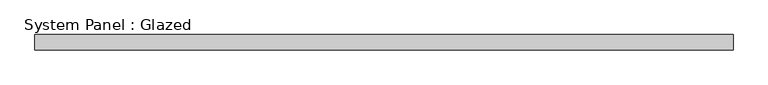
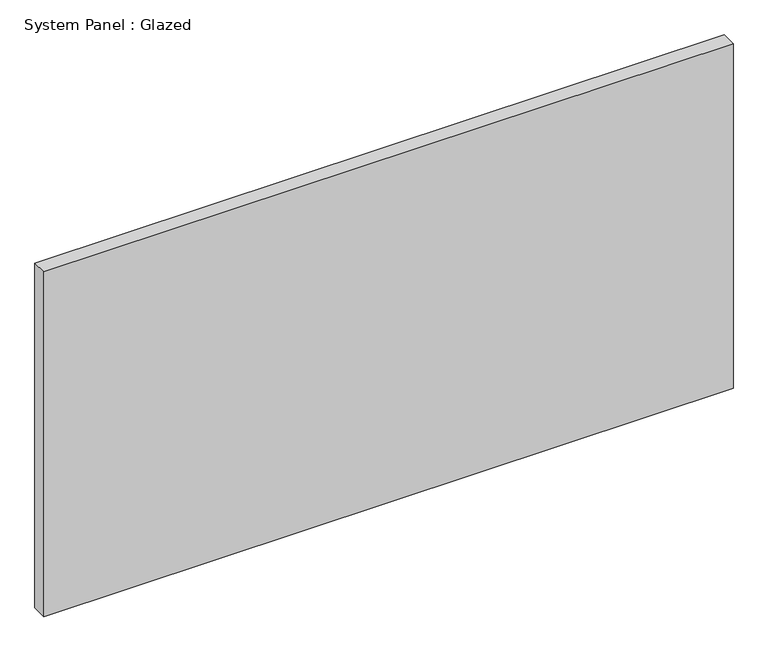
"""IFC4 building model written with IfcOpenShell, lengths in millimetres: plate geometry, System Panel : Glazed."""

from ifc_helpers import new_model, si_unit, origin, origin_with_axes, place, context, project, spatial, polyline, outline, extrude, source, transform, mapped, element, save


def system_panel_glazed_d447efa8(model_context):
    return source(origin(), model_context, "Body", "SweptSolid", [
        extrude(outline(polyline([(576.624914, 19.05), (-576.624914, 19.05), (-576.624914, 44.45), (576.624914, 44.45), (576.624914, 19.05)])), origin_with_axes(), (0.0, 0.0, 1.0), 609.6),
    ])


if __name__ == "__main__":
    model = new_model("IFC4")
    model_context = context("Model", 3, world=origin())
    ifc_project = project(units=[si_unit("LENGTHUNIT", "METRE", prefix="MILLI")], contexts=[model_context])
    site = spatial("IfcSite", under=ifc_project)
    building = spatial("IfcBuilding", under=site)
    placement = place(None, origin())
    system_panel_glazed_shape = system_panel_glazed_d447efa8(model_context)
    element("IfcPlate", 1, ObjectType="System Panel : Glazed", at=placement, inside=building, context=model_context, shape_type="MappedRepresentation", body=[
        mapped(system_panel_glazed_shape, transform((0.0, 0.0, 0.0), x_axis=(1.0, 0.0, 0.0), y_axis=(0.0, 1.0, 0.0), z_axis=(0.0, 0.0, 1.0))),
    ])
    save(model, "model.ifc")

# Revit data of these elements
# Element 1 (IfcPlate, "System Panel : Glazed")
#   Materials on its faces: "Glass"
# Materials
#   "Glass": class "Glass", colour RGB 0 128 192, transparency 0.75
